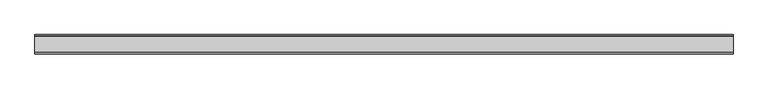
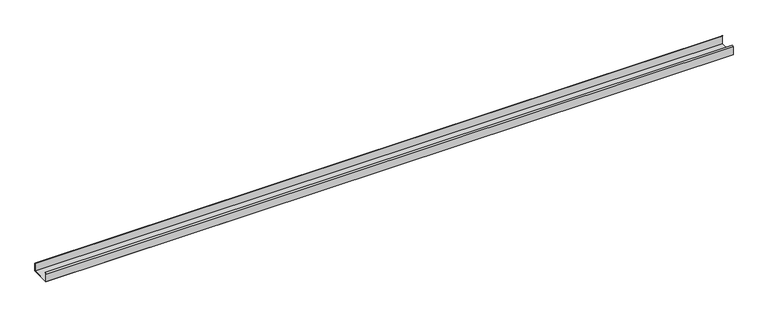
"""IFC4 building model written with IfcOpenShell, lengths in millimetres: proxy geometry, Generic Models 7:Generic Models 1:1:Generic Models 1:1 : Generic Models 7:Generic Models 1:337419:5 : Generic Models 7:Generic Models 1:1:Generic Models 1:1 : Generic Models 7:Generic Models 1:337419:306201."""

import ifcopenshell
import ifcopenshell.guid

model = None  # the IFC model being written
_history = None  # IfcOwnerHistory: only IFC2X3 demands one
_inside = {}  # id of a spatial element -> (the spatial element, [elements in it])
_under = {}  # id of a project, library or spatial element -> (it, [spatial elements below it])
_declared = {}  # id of a project -> (the project, [libraries it declares])
_typed = {}  # id of a type object -> (the type object, [elements of that type])
_made_of = {}  # id of a material, layer set ... -> (it, [elements and type objects made of it])


def new_model(schema):
    """Start an empty IFC model of exactly this schema.

    Asked for "IFC4X3", IfcOpenShell would pick the latest addendum, in which some entities
    have other attributes; the version numbers below select the first issue.
    IFC2X3 requires an IfcOwnerHistory on every rooted entity: one is made here for all.
    """
    global model, _history
    if schema == "IFC4X3":
        model = ifcopenshell.file(schema_version=(4, 3, 0, 0))
    else:
        model = ifcopenshell.file(schema=schema)
    _inside.clear()
    _under.clear()
    _declared.clear()
    _typed.clear()
    _made_of.clear()
    _history = None
    if model.schema == "IFC2X3":
        org = make("IfcOrganization", Name="unknown")
        user = make(
            "IfcPersonAndOrganization",
            ThePerson=make("IfcPerson", FamilyName="unknown"),
            TheOrganization=org,
        )
        app = make(
            "IfcApplication",
            ApplicationDeveloper=org,
            Version="unknown",
            ApplicationFullName="unknown",
            ApplicationIdentifier="unknown",
        )
        _history = make(
            "IfcOwnerHistory",
            OwningUser=user,
            OwningApplication=app,
            ChangeAction="ADDED",
            CreationDate=0,
        )
    return model


def make(cls, **values):
    """One entity of the class cls with the attributes given. An attribute that is None is left unset."""
    return model.create_entity(
        cls, **{name: value for name, value in values.items() if value is not None}
    )


def rooted(cls, **values):
    """An entity with a GlobalId (a new one), such as an element, a storey or a relation."""
    return make(cls, GlobalId=ifcopenshell.guid.new(), OwnerHistory=_history, **values)


def si_unit(unit_type, name, prefix=None):
    """IfcSIUnit, for example si_unit("LENGTHUNIT", "METRE", prefix="MILLI")."""
    return make("IfcSIUnit", UnitType=unit_type, Prefix=prefix, Name=name)


def assignment(units):
    """IfcUnitAssignment: the units of a project."""
    return None if units is None else make("IfcUnitAssignment", Units=units)


def point(xyz):
    """IfcCartesianPoint."""
    return None if xyz is None else make("IfcCartesianPoint", Coordinates=xyz)


def direction(xyz):
    """IfcDirection."""
    return None if xyz is None else make("IfcDirection", DirectionRatios=xyz)


def frame(location, z_axis=None, x_axis=None):
    """IfcAxis2Placement3D, a coordinate frame: its origin and axes. An axis left out is left unset."""
    return make(
        "IfcAxis2Placement3D",
        Location=point(location),
        Axis=direction(z_axis),
        RefDirection=direction(x_axis),
    )


def origin():
    """The frame at (0, 0, 0) with its axes left unset."""
    return frame((0.0, 0.0, 0.0))


def place(relative_to, where):
    """IfcLocalPlacement: puts the frame where relative to a parent placement (None: the world)."""
    return make(
        "IfcLocalPlacement", PlacementRelTo=relative_to, RelativePlacement=where
    )


def context(
    kind, dimensions, precision=None, world=None, true_north=None, identifier=None
):
    """IfcGeometricRepresentationContext, for example the 3D "Model" context."""
    return make(
        "IfcGeometricRepresentationContext",
        ContextIdentifier=identifier,
        ContextType=kind,
        CoordinateSpaceDimension=dimensions,
        Precision=precision,
        WorldCoordinateSystem=world,
        TrueNorth=true_north,
    )


def project(units=None, contexts=None):
    """IfcProject with its units and contexts."""
    return rooted(
        "IfcProject",
        Name="project",
        RepresentationContexts=contexts,
        UnitsInContext=assignment(units),
    )


def spatial(cls, under=None, at=None, **own):
    """A site, building, storey or space (cls), placed at a placement, below another one or the project."""
    s = rooted(cls, ObjectPlacement=at, **own)
    if under is not None:
        _under.setdefault(under.id(), (under, []))[1].append(s)
    return s


def polyline(points):
    """IfcPolyline through the points."""
    return make("IfcPolyline", Points=[point(p) for p in points])


def outline(outer, holes=None, kind="AREA"):
    """IfcArbitraryClosedProfileDef: a profile drawn as a closed curve; with holes, ...WithVoids."""
    if holes is None:
        return make("IfcArbitraryClosedProfileDef", ProfileType=kind, OuterCurve=outer)
    return make(
        "IfcArbitraryProfileDefWithVoids",
        ProfileType=kind,
        OuterCurve=outer,
        InnerCurves=holes,
    )


def extrude(swept, where, along, depth):
    """IfcExtrudedAreaSolid: the profile swept, set in the frame where, extruded along a direction by depth."""
    return make(
        "IfcExtrudedAreaSolid",
        SweptArea=swept,
        Position=where,
        ExtrudedDirection=direction(along),
        Depth=depth,
    )


def shape(context_of_items, identifier, shape_type, items):
    """IfcShapeRepresentation: the items that make up one representation, for example the "Body"."""
    return make(
        "IfcShapeRepresentation",
        ContextOfItems=context_of_items,
        RepresentationIdentifier=identifier,
        RepresentationType=shape_type,
        Items=items,
    )


def source(mapping_origin, context_of_items, identifier, shape_type, items):
    """IfcRepresentationMap: a shape defined once, which mapped items show again and again."""
    return make(
        "IfcRepresentationMap",
        MappingOrigin=mapping_origin,
        MappedRepresentation=shape(context_of_items, identifier, shape_type, items),
    )


def transform(
    local_origin,
    x_axis=None,
    y_axis=None,
    z_axis=None,
    scale=None,
    scale2=None,
    scale3=None,
    uniform=True,
):
    """IfcCartesianTransformationOperator3D, or its non-uniform kind. x_axis, y_axis, z_axis: its Axis1, 2, 3."""
    if uniform:
        return make(
            "IfcCartesianTransformationOperator3D",
            Axis1=direction(x_axis),
            Axis2=direction(y_axis),
            LocalOrigin=point(local_origin),
            Scale=scale,
            Axis3=direction(z_axis),
        )
    return make(
        "IfcCartesianTransformationOperator3DnonUniform",
        Axis1=direction(x_axis),
        Axis2=direction(y_axis),
        LocalOrigin=point(local_origin),
        Scale=scale,
        Axis3=direction(z_axis),
        Scale2=scale2,
        Scale3=scale3,
    )


def mapped(mapping_source, mapping_target):
    """IfcMappedItem: shows the shape of a source again, moved by a transform."""
    return make(
        "IfcMappedItem", MappingSource=mapping_source, MappingTarget=mapping_target
    )


def made_of(thing, what):
    """Note that an element or type object is made of a material, layer set ...; save() writes the relation."""
    if what is not None:
        _made_of.setdefault(what.id(), (what, []))[1].append(thing)
    return thing


def element(
    cls,
    number,
    at=None,
    inside=None,
    cuts=None,
    type_object=None,
    material=None,
    context=None,
    identifier="Body",
    shape_type=None,
    held_by="IfcProductDefinitionShape",
    body=None,
    shapes=None,
    **own,
):
    """One element of the class cls, such as IfcWall. Its Tag is "e" and its number.

    at: its placement. inside: the storey or other place that contains it. cuts: it is an
    opening in that element (IfcRelVoidsElement). A single representation is given by context,
    identifier, shape_type and body (its items); several are given by shapes. held_by: the class
    of the entity that holds the representations. save() writes the other relations.
    """
    e = rooted(cls, Tag="e%d" % number, ObjectPlacement=at, **own)
    if body is not None:
        shapes = [shape(context, identifier, shape_type, body)]
    if shapes is not None:
        e.Representation = make(held_by, Representations=shapes)
    if inside is not None:
        _inside.setdefault(inside.id(), (inside, []))[1].append(e)
    if cuts is not None:
        rooted(
            "IfcRelVoidsElement", RelatingBuildingElement=cuts, RelatedOpeningElement=e
        )
    if type_object is not None:
        _typed.setdefault(type_object.id(), (type_object, []))[1].append(e)
    return made_of(e, material)


def aggregate(whole, parts):
    """IfcRelAggregates: a whole, such as a stair, and the parts it consists of."""
    return rooted("IfcRelAggregates", RelatingObject=whole, RelatedObjects=parts)


def save(model, path):
    """Write the relations noted so far, then the file.

    IfcRelAggregates (storeys below a building ...), IfcRelContainedInSpatialStructure (elements
    in a storey), IfcRelDefinesByType, IfcRelAssociatesMaterial and IfcRelDeclares: one each for
    every whole, place, type object, material and project.
    """
    for whole, parts in _under.values():
        aggregate(whole, parts)
    for where, things in _inside.values():
        rooted(
            "IfcRelContainedInSpatialStructure",
            RelatedElements=things,
            RelatingStructure=where,
        )
    for kind, things in _typed.values():
        rooted("IfcRelDefinesByType", RelatedObjects=things, RelatingType=kind)
    for what, things in _made_of.values():
        rooted("IfcRelAssociatesMaterial", RelatedObjects=things, RelatingMaterial=what)
    for by, libraries in _declared.values():
        rooted("IfcRelDeclares", RelatingContext=by, RelatedDefinitions=libraries)
    model.write(path)


def generic_models_29d2b25b(model_context):
    return source(origin(), model_context, "Body", "SweptSolid", [
        extrude(outline(polyline([(-578797.4913841, 3617.9125), (-579000.6913841, 3617.9125), (-579000.6913841, 3706.8125), (-578986.0982375, 3719.057604), (-578984.3124931, 3716.9294367), (-578997.9132591, 3705.517039), (-578997.9132591, 3620.690625), (-578800.2695091, 3620.690625), (-578800.2695091, 3705.517039), (-578813.8702751, 3716.9294367), (-578812.0845307, 3719.057604), (-578797.4913841, 3706.8125), (-578797.4913841, 3617.9125)])), frame((588867.6367239, 0.0, 0.0), z_axis=(1.0, 0.0, 0.0), x_axis=(0.0, 1.0, 0.0)), (0.0, 0.0, 1.0), 7315.2),
    ])


if __name__ == "__main__":
    model = new_model("IFC4")
    model_context = context("Model", 3, world=origin())
    ifc_project = project(units=[si_unit("LENGTHUNIT", "METRE", prefix="MILLI")], contexts=[model_context])
    site = spatial("IfcSite", under=ifc_project)
    building = spatial("IfcBuilding", under=site)
    placement = place(None, origin())
    generic_models_shape = generic_models_29d2b25b(model_context)
    element("IfcBuildingElementProxy", 1, Name="Generic Models 7:Generic Models 1:1:Generic Models 1:1 : Generic Models 7:Generic Models 1:337419:5 : Generic Models 7:Generic Models 1:1:Generic Models 1:1 : Generic Models 7:Generic Models 1:337419:306201", ObjectType="Generic Models 7:Generic Models 1:1:Generic Models 1:1 : Generic Models 7:Generic Models 1:337419:5 : Generic Models 7:Generic Models 1:1:Generic Models 1:1 : Generic Models 7:Generic Models 1:337419:306201", at=placement, inside=building, context=model_context, shape_type="MappedRepresentation", body=[
        mapped(generic_models_shape, transform((0.0, 0.0, 0.0), x_axis=(1.0, 0.0, 0.0), y_axis=(0.0, 1.0, 0.0), z_axis=(0.0, 0.0, 1.0))),
    ])
    save(model, "model.ifc")

# Revit data of these elements
# Type "Generic Models 7:Generic Models 1:1:Generic Models 1:1 : Generic Models 7:Generic Models 1:337419:5 : Generic Models 7:Generic Models 1:1:Generic Models 1:1 : Generic Models 7:Generic Models 1:337419:306201"
#   NameOverride = "Generic Models 7:Generic Models 1:1:Generic Models 1:1 : Generic Models 7:Generic Models 1:337419:306201"
#   ObjectTypeOverride = "Generic Models 1:1 : Generic Models 7:Generic Models 1:337419"
#   Reference = "Generic Models 1"
#   Tag = "306201"
# Element 1 (IfcBuildingElementProxy, "Generic Models 7:Generic Models 1:1:Generic Models 1:1 : Generic Models 7:Generic Models 1:337419:5 : Generic Models 7:Generic Models 1:1:Generic Models 1:1 : Generic Models 7:Generic Models 1:337419:306201")
#   Materials on its faces: "CEE' SECTION (8.0x3.5C - SEE STRUCT. DWGS)"
# Materials
#   "CEE' SECTION (8.0x3.5C - SEE STRUCT. DWGS)": class "Unassigned", colour RGB 210 209 208, transparency 0, Keynote = "M05121300.02", Cost = 0
